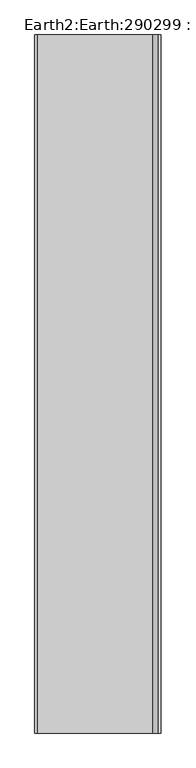
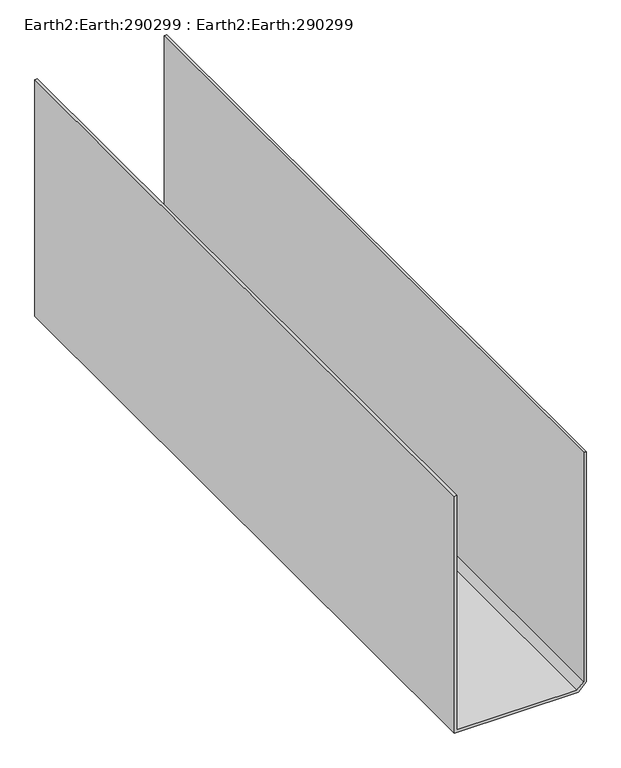
"""IFC4 building model written with IfcOpenShell, lengths in millimetres: proxy geometry, Earth2:Earth:290299 : Earth2:Earth:290299."""

from ifc_helpers import new_model, si_unit, frame, origin, place, context, project, spatial, polyline, outline, extrude, source, transform, mapped, element, save


def earth2_earth_290299_earth2_earth_290299_4e8750fb(model_context):
    return source(origin(), model_context, "Body", "SweptSolid", [
        extrude(outline(polyline([(33309.014262, -5280.5615232), (32620.9902343, -5280.5615232), (32620.9902343, -4940.2057359), (32643.1028304, -4918.0931398), (33313.1445312, -4918.0931398), (33313.1445312, -4925.0931398), (32646.0023253, -4925.0931398), (32627.9902343, -4943.1052309), (32627.9902343, -5273.5615232), (33310.3609003, -5273.5615232), (33309.014262, -5280.5615232)])), frame((0.0, 7460.4857132, 0.0), z_axis=(0.0, 1.0, 0.0), x_axis=(0.0, 0.0, 1.0)), (0.0, 0.0, 1.0), 2000.0),
    ])


if __name__ == "__main__":
    model = new_model("IFC4")
    model_context = context("Model", 3, world=origin())
    ifc_project = project(units=[si_unit("LENGTHUNIT", "METRE", prefix="MILLI")], contexts=[model_context])
    site = spatial("IfcSite", under=ifc_project)
    building = spatial("IfcBuilding", under=site)
    placement = place(None, origin())
    earth2_earth_290299_earth2_earth_290299_shape = earth2_earth_290299_earth2_earth_290299_4e8750fb(model_context)
    element("IfcBuildingElementProxy", 1, Name="Earth2:Earth:290299 : Earth2:Earth:290299", ObjectType="Earth2:Earth:290299 : Earth2:Earth:290299", at=placement, inside=building, context=model_context, shape_type="MappedRepresentation", body=[
        mapped(earth2_earth_290299_earth2_earth_290299_shape, transform((0.0, 0.0, 0.0), x_axis=(1.0, 0.0, 0.0), y_axis=(0.0, 1.0, 0.0), z_axis=(0.0, 0.0, 1.0))),
    ])
    save(model, "model.ifc")

# Revit data of these elements
# Type "Earth2:Earth:290299 : Earth2:Earth:290299"
#   NameOverride = "Earth2:Earth:290299"
#   ObjectTypeOverride = "Earth2:Earth"
#   Reference = "Earth"
#   Category = "Generic Models"
#   Tag = "290299"
# Element 1 (IfcBuildingElementProxy, "Earth2:Earth:290299 : Earth2:Earth:290299")
#   Materials on its faces: "WATERPROOF FIBER GLASS PLANTER LINER"
# Materials
#   "WATERPROOF FIBER GLASS PLANTER LINER": class "Unassigned", colour RGB 221 220 200, transparency 0, Cost = 0
